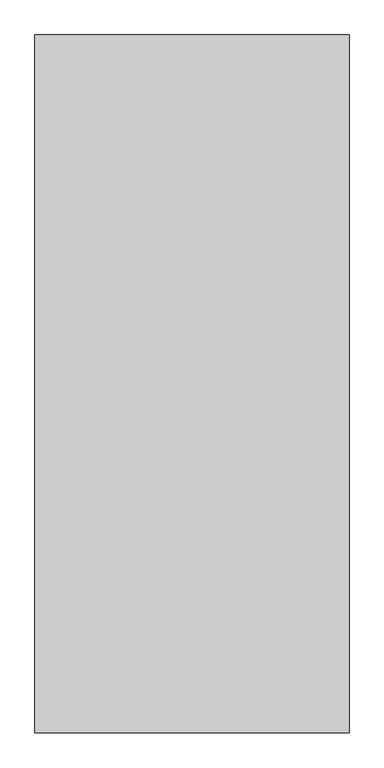
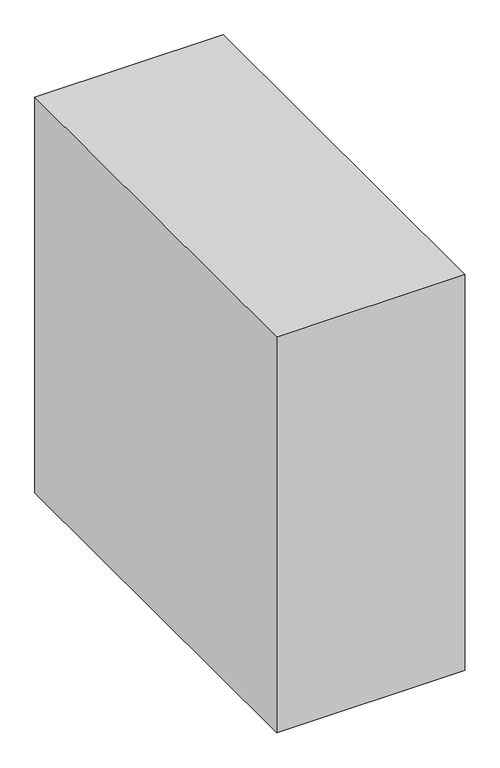
"""IFC4 building model written with IfcOpenShell, lengths in millimetres: proxy geometry, Space Planning Box_hec : Space Planning Box_hec."""

import ifcopenshell
import ifcopenshell.guid

model = None  # the IFC model being written
_history = None  # IfcOwnerHistory: only IFC2X3 demands one
_inside = {}  # id of a spatial element -> (the spatial element, [elements in it])
_under = {}  # id of a project, library or spatial element -> (it, [spatial elements below it])
_declared = {}  # id of a project -> (the project, [libraries it declares])
_typed = {}  # id of a type object -> (the type object, [elements of that type])
_made_of = {}  # id of a material, layer set ... -> (it, [elements and type objects made of it])


def new_model(schema):
    """Start an empty IFC model of exactly this schema.

    Asked for "IFC4X3", IfcOpenShell would pick the latest addendum, in which some entities
    have other attributes; the version numbers below select the first issue.
    IFC2X3 requires an IfcOwnerHistory on every rooted entity: one is made here for all.
    """
    global model, _history
    if schema == "IFC4X3":
        model = ifcopenshell.file(schema_version=(4, 3, 0, 0))
    else:
        model = ifcopenshell.file(schema=schema)
    _inside.clear()
    _under.clear()
    _declared.clear()
    _typed.clear()
    _made_of.clear()
    _history = None
    if model.schema == "IFC2X3":
        org = make("IfcOrganization", Name="unknown")
        user = make(
            "IfcPersonAndOrganization",
            ThePerson=make("IfcPerson", FamilyName="unknown"),
            TheOrganization=org,
        )
        app = make(
            "IfcApplication",
            ApplicationDeveloper=org,
            Version="unknown",
            ApplicationFullName="unknown",
            ApplicationIdentifier="unknown",
        )
        _history = make(
            "IfcOwnerHistory",
            OwningUser=user,
            OwningApplication=app,
            ChangeAction="ADDED",
            CreationDate=0,
        )
    return model


def make(cls, **values):
    """One entity of the class cls with the attributes given. An attribute that is None is left unset."""
    return model.create_entity(
        cls, **{name: value for name, value in values.items() if value is not None}
    )


def rooted(cls, **values):
    """An entity with a GlobalId (a new one), such as an element, a storey or a relation."""
    return make(cls, GlobalId=ifcopenshell.guid.new(), OwnerHistory=_history, **values)


def si_unit(unit_type, name, prefix=None):
    """IfcSIUnit, for example si_unit("LENGTHUNIT", "METRE", prefix="MILLI")."""
    return make("IfcSIUnit", UnitType=unit_type, Prefix=prefix, Name=name)


def assignment(units):
    """IfcUnitAssignment: the units of a project."""
    return None if units is None else make("IfcUnitAssignment", Units=units)


def point(xyz):
    """IfcCartesianPoint."""
    return None if xyz is None else make("IfcCartesianPoint", Coordinates=xyz)


def direction(xyz):
    """IfcDirection."""
    return None if xyz is None else make("IfcDirection", DirectionRatios=xyz)


def frame(location, z_axis=None, x_axis=None):
    """IfcAxis2Placement3D, a coordinate frame: its origin and axes. An axis left out is left unset."""
    return make(
        "IfcAxis2Placement3D",
        Location=point(location),
        Axis=direction(z_axis),
        RefDirection=direction(x_axis),
    )


def origin():
    """The frame at (0, 0, 0) with its axes left unset."""
    return frame((0.0, 0.0, 0.0))


def origin_with_axes():
    """The frame at (0, 0, 0) with the z axis (0, 0, 1) and the x axis (1, 0, 0) written out."""
    return frame((0.0, 0.0, 0.0), z_axis=(0.0, 0.0, 1.0), x_axis=(1.0, 0.0, 0.0))


def place(relative_to, where):
    """IfcLocalPlacement: puts the frame where relative to a parent placement (None: the world)."""
    return make(
        "IfcLocalPlacement", PlacementRelTo=relative_to, RelativePlacement=where
    )


def context(
    kind, dimensions, precision=None, world=None, true_north=None, identifier=None
):
    """IfcGeometricRepresentationContext, for example the 3D "Model" context."""
    return make(
        "IfcGeometricRepresentationContext",
        ContextIdentifier=identifier,
        ContextType=kind,
        CoordinateSpaceDimension=dimensions,
        Precision=precision,
        WorldCoordinateSystem=world,
        TrueNorth=true_north,
    )


def project(units=None, contexts=None):
    """IfcProject with its units and contexts."""
    return rooted(
        "IfcProject",
        Name="project",
        RepresentationContexts=contexts,
        UnitsInContext=assignment(units),
    )


def spatial(cls, under=None, at=None, **own):
    """A site, building, storey or space (cls), placed at a placement, below another one or the project."""
    s = rooted(cls, ObjectPlacement=at, **own)
    if under is not None:
        _under.setdefault(under.id(), (under, []))[1].append(s)
    return s


def polyline(points):
    """IfcPolyline through the points."""
    return make("IfcPolyline", Points=[point(p) for p in points])


def outline(outer, holes=None, kind="AREA"):
    """IfcArbitraryClosedProfileDef: a profile drawn as a closed curve; with holes, ...WithVoids."""
    if holes is None:
        return make("IfcArbitraryClosedProfileDef", ProfileType=kind, OuterCurve=outer)
    return make(
        "IfcArbitraryProfileDefWithVoids",
        ProfileType=kind,
        OuterCurve=outer,
        InnerCurves=holes,
    )


def extrude(swept, where, along, depth):
    """IfcExtrudedAreaSolid: the profile swept, set in the frame where, extruded along a direction by depth."""
    return make(
        "IfcExtrudedAreaSolid",
        SweptArea=swept,
        Position=where,
        ExtrudedDirection=direction(along),
        Depth=depth,
    )


def shape(context_of_items, identifier, shape_type, items):
    """IfcShapeRepresentation: the items that make up one representation, for example the "Body"."""
    return make(
        "IfcShapeRepresentation",
        ContextOfItems=context_of_items,
        RepresentationIdentifier=identifier,
        RepresentationType=shape_type,
        Items=items,
    )


def source(mapping_origin, context_of_items, identifier, shape_type, items):
    """IfcRepresentationMap: a shape defined once, which mapped items show again and again."""
    return make(
        "IfcRepresentationMap",
        MappingOrigin=mapping_origin,
        MappedRepresentation=shape(context_of_items, identifier, shape_type, items),
    )


def transform(
    local_origin,
    x_axis=None,
    y_axis=None,
    z_axis=None,
    scale=None,
    scale2=None,
    scale3=None,
    uniform=True,
):
    """IfcCartesianTransformationOperator3D, or its non-uniform kind. x_axis, y_axis, z_axis: its Axis1, 2, 3."""
    if uniform:
        return make(
            "IfcCartesianTransformationOperator3D",
            Axis1=direction(x_axis),
            Axis2=direction(y_axis),
            LocalOrigin=point(local_origin),
            Scale=scale,
            Axis3=direction(z_axis),
        )
    return make(
        "IfcCartesianTransformationOperator3DnonUniform",
        Axis1=direction(x_axis),
        Axis2=direction(y_axis),
        LocalOrigin=point(local_origin),
        Scale=scale,
        Axis3=direction(z_axis),
        Scale2=scale2,
        Scale3=scale3,
    )


def mapped(mapping_source, mapping_target):
    """IfcMappedItem: shows the shape of a source again, moved by a transform."""
    return make(
        "IfcMappedItem", MappingSource=mapping_source, MappingTarget=mapping_target
    )


def made_of(thing, what):
    """Note that an element or type object is made of a material, layer set ...; save() writes the relation."""
    if what is not None:
        _made_of.setdefault(what.id(), (what, []))[1].append(thing)
    return thing


def element(
    cls,
    number,
    at=None,
    inside=None,
    cuts=None,
    type_object=None,
    material=None,
    context=None,
    identifier="Body",
    shape_type=None,
    held_by="IfcProductDefinitionShape",
    body=None,
    shapes=None,
    **own,
):
    """One element of the class cls, such as IfcWall. Its Tag is "e" and its number.

    at: its placement. inside: the storey or other place that contains it. cuts: it is an
    opening in that element (IfcRelVoidsElement). A single representation is given by context,
    identifier, shape_type and body (its items); several are given by shapes. held_by: the class
    of the entity that holds the representations. save() writes the other relations.
    """
    e = rooted(cls, Tag="e%d" % number, ObjectPlacement=at, **own)
    if body is not None:
        shapes = [shape(context, identifier, shape_type, body)]
    if shapes is not None:
        e.Representation = make(held_by, Representations=shapes)
    if inside is not None:
        _inside.setdefault(inside.id(), (inside, []))[1].append(e)
    if cuts is not None:
        rooted(
            "IfcRelVoidsElement", RelatingBuildingElement=cuts, RelatedOpeningElement=e
        )
    if type_object is not None:
        _typed.setdefault(type_object.id(), (type_object, []))[1].append(e)
    return made_of(e, material)


def aggregate(whole, parts):
    """IfcRelAggregates: a whole, such as a stair, and the parts it consists of."""
    return rooted("IfcRelAggregates", RelatingObject=whole, RelatedObjects=parts)


def save(model, path):
    """Write the relations noted so far, then the file.

    IfcRelAggregates (storeys below a building ...), IfcRelContainedInSpatialStructure (elements
    in a storey), IfcRelDefinesByType, IfcRelAssociatesMaterial and IfcRelDeclares: one each for
    every whole, place, type object, material and project.
    """
    for whole, parts in _under.values():
        aggregate(whole, parts)
    for where, things in _inside.values():
        rooted(
            "IfcRelContainedInSpatialStructure",
            RelatedElements=things,
            RelatingStructure=where,
        )
    for kind, things in _typed.values():
        rooted("IfcRelDefinesByType", RelatedObjects=things, RelatingType=kind)
    for what, things in _made_of.values():
        rooted("IfcRelAssociatesMaterial", RelatedObjects=things, RelatingMaterial=what)
    for by, libraries in _declared.values():
        rooted("IfcRelDeclares", RelatingContext=by, RelatedDefinitions=libraries)
    model.write(path)


def generic_models_5634f436(model_context):
    return source(origin(), model_context, "Body", "SweptSolid", [
        extrude(outline(polyline([(1350.0, 3000.0), (1350.0, -3000.0), (-1350.0, -3000.0), (-1350.0, 3000.0), (1350.0, 3000.0)])), origin_with_axes(), (0.0, 0.0, 1.0), 6000.0),
    ])


if __name__ == "__main__":
    model = new_model("IFC4")
    model_context = context("Model", 3, world=origin())
    ifc_project = project(units=[si_unit("LENGTHUNIT", "METRE", prefix="MILLI")], contexts=[model_context])
    site = spatial("IfcSite", under=ifc_project)
    building = spatial("IfcBuilding", under=site)
    placement = place(None, origin())
    generic_models_shape = generic_models_5634f436(model_context)
    element("IfcBuildingElementProxy", 1, Name="Space Planning Box_hec : Space Planning Box_hec", ObjectType="Space Planning Box_hec : Space Planning Box_hec", at=placement, inside=building, context=model_context, shape_type="MappedRepresentation", body=[
        mapped(generic_models_shape, transform((0.0, 0.0, 0.0), x_axis=(1.0, 0.0, 0.0), y_axis=(0.0, 1.0, 0.0), z_axis=(0.0, 0.0, 1.0))),
    ])
    save(model, "model.ifc")

# Revit data of these elements
# Type "Space Planning Box_hec : Space Planning Box_hec"
#   Type Comments = "..."
#   Room Name [instance default] = "?"
#   Interior Finish [instance default] = ""
#   Exterior Finish [instance default] = ""
#   Department [instance default] = ""
#   Assembly Code = "..."
#   Width [instance default] = 1524 mm
#   Program Area [instance default] = 0.00 m²
#   Length [instance default] = 1524 mm
#   Height [instance default] = 1524 mm
#   Area [instance default] = 2.32258 m²
#   Fill Color [instance default] = Cyan
#   Default Elevation = 0
# Element 1 (IfcBuildingElementProxy, "Space Planning Box_hec : Space Planning Box_hec")
#   Room Name = "Duct Shaft"
#   Interior Finish = "NA"
#   Exterior Finish = "EF1"
#   Department = "HV"
#   Width = 2700 mm
#   Program Area = 16.20 m²
#   Length = 6000 mm
#   Height = 6000 mm
#   Area = 16.20 m²
#   Fill Color = Pink
#   Materials on its faces: "Pink"
# Materials
#   "Cyan": class "Generic", colour RGB 0 255 255, transparency 0.2, Cost = 0
#   "Pink": class "Generic", colour RGB 255 105 180, transparency 0.2, Cost = 0
